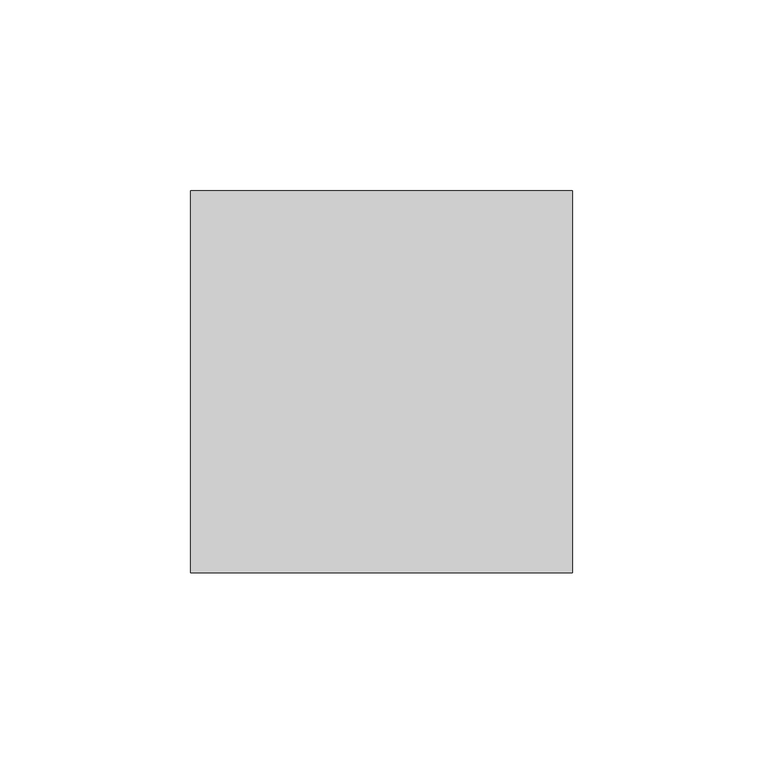
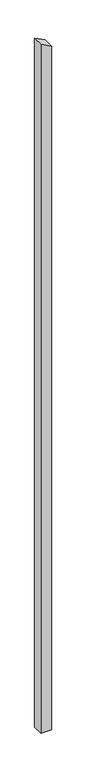
"""IFC4 building model written with IfcOpenShell, lengths in millimetres: column geometry, Holzstütze 159306 : Holzstütze 159306."""

from ifc_helpers import new_model, si_unit, frame, origin, place, context, project, spatial, polyline, outline, extrude, source, transform, mapped, element, save


def column_070c94f2(model_context):
    return source(origin(), model_context, "Body", "SweptSolid", [
        extrude(outline(polyline([(-500.0, 174197.7593015), (-500.0, 174297.7593015), (6345.7118258, 174297.7593015), (6396.6643707, 174197.7593015), (-500.0, 174197.7593015)])), frame((0.0, 39349.3988814, 0.0), z_axis=(0.0, 1.0, 0.0), x_axis=(0.0, 0.0, 1.0)), (0.0, 0.0, 1.0), 100.0),
    ])


if __name__ == "__main__":
    model = new_model("IFC4")
    model_context = context("Model", 3, world=origin())
    ifc_project = project(units=[si_unit("LENGTHUNIT", "METRE", prefix="MILLI")], contexts=[model_context])
    site = spatial("IfcSite", under=ifc_project)
    building = spatial("IfcBuilding", under=site)
    placement = place(None, origin())
    column_shape = column_070c94f2(model_context)
    element("IfcColumn", 1, ObjectType="Holzstütze 159306 : Holzstütze 159306", at=placement, inside=building, context=model_context, shape_type="MappedRepresentation", body=[
        mapped(column_shape, transform((0.0, 0.0, 0.0), x_axis=(1.0, 0.0, 0.0), y_axis=(0.0, 1.0, 0.0), z_axis=(0.0, 0.0, 1.0))),
    ])
    save(model, "model.ifc")

# Revit data of these elements
# Type "Holzstütze 159306 : Holzstütze 159306"
#   Abrechnungsart = "m"
#   Allright_Bauteil_ID = "0152St 0000143477"
#   Bezeichnung = "Holzstütze"
#   Codetext = "ST-HOLZ\\"
#   Gewerk = "Zimmer- und Holzbauarbeiten"
#   Material = "Holz"
#   Objektname = "Stütze"
#   NameOverride = "Holzstütze"
#   Reference = "Holzstütze"
#   Status = "NEW"
#   ThermalTransmittance = 0.0000 BTU/(h·ft²·°F)
#   Roll = 0.00°
#   Slope = 0.00°
#   2D Interaktion = yes
#   IsExternal = yes
#   LoadBearing = yes
# Element 1 (IfcColumn, "Holzstütze 159306 : Holzstütze 159306")
#   Materials on its faces: "holzschalung"
# Materials
#   "holzschalung": class "Unassigned", colour RGB 128 128 128, transparency 0
